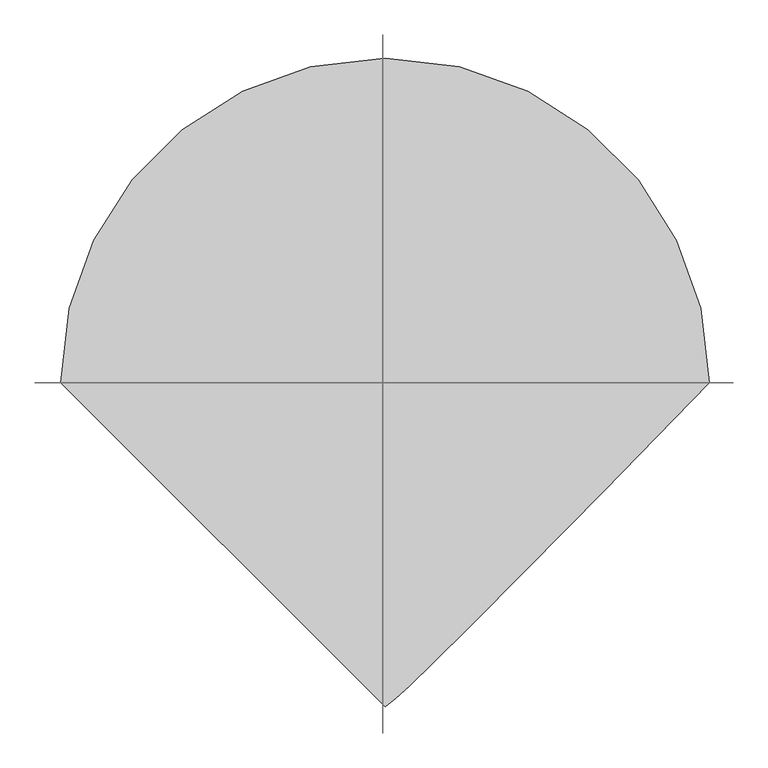
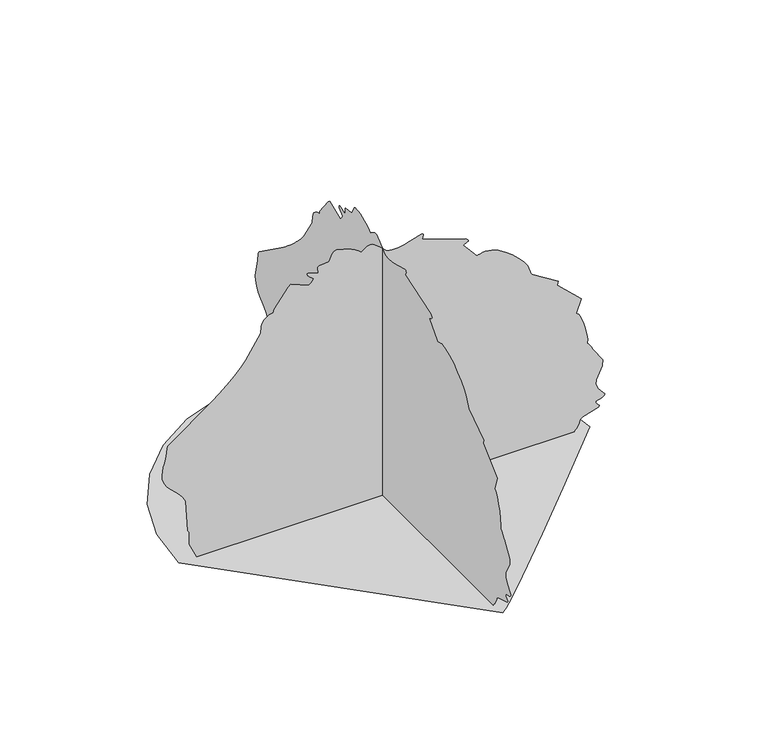
"""IFC4 building model written with IfcOpenShell, lengths in millimetres: proxy geometry, holly 26750 : holly 26750."""

from ifc_helpers import new_model, si_unit, origin, place, context, project, spatial, triangles, source, transform, mapped, element, save


def entourage_ccbe6d7c(model_context):
    return source(origin(), model_context, "Body", "Tessellation", [
        triangles([(-948.1489574, 0.0, 0.0001584), (-923.0842083, 217.2530545, 0.0001584), (-851.6949612, 416.7657311, 0.0001584), (-739.7012884, 592.8207553, 0.0001584), (-592.8207553, 739.7012884, 0.0001584), (-416.7657311, 851.6949612, 0.0001584), (-217.2530545, 923.0816648, 0.0001584), (4.14e-05, 948.1489574, 0.0001584), (217.2530545, 923.0842083, 0.0001584), (416.7657311, 851.6949612, 0.0001584), (592.8207553, 739.7012884, 0.0001584), (739.7012884, 592.8207553, 0.0001584), (851.6949612, 416.7657311, 0.0001584), (923.0816648, 217.2530545, 0.0001584), (948.1489574, -8.29e-05, 0.0001584), (640.0215443, -316.0623576, 0.0001584), (411.5917374, -548.7669763, 0.0001584), (249.5753185, -712.0026157, 0.0001584), (140.6913579, -819.6655935, 0.0001584), (71.6559369, -885.64972, 0.0001584), (29.1863771, -923.8462257, 0.0001584), (-0.0001243, -948.1489574, 0.0001584), (-7.5086714, 195.1763861, 1267.2389282), (-7.5086714, 179.2483067, 1263.2994884), (-7.5086714, 162.0304078, 1257.8307816), (-7.5086714, 144.4787539, 1250.7569401), (-7.5086714, 127.5514259, 1242.0092182), (-7.5086714, 112.2047518, 1231.5139286), (-7.5086714, 99.3960405, 1219.1973839), (-7.5086714, 96.3241623, 1220.6731659), (-7.5086714, 91.1522123, 1224.4323841), (-7.5086714, 84.5334848, 1229.4921043), (-7.5086714, 77.1194751, 1234.8564571), (-7.5086714, 69.5642495, 1239.5377121), (-7.5086714, 62.5195578, 1242.5399998), (-7.5086714, 56.6381899, 1242.880386), (-7.5086714, 48.1497636, 1241.0642178), (-7.5086714, 38.0075433, 1235.3112259), (-7.5086714, 26.6616175, 1226.6954727), (-7.5086714, 14.5605495, 1216.2942181), (-7.5086714, 2.1549868, 1205.1816696), (-7.5086714, -10.1063292, 1194.4323984), (-7.5086714, -21.7735642, 1185.1233009), (-7.5086714, -44.9310738, 1181.1406225), (-7.5086714, -71.2939859, 1182.9871668), (-7.5086714, -98.7844045, 1188.6996088), (-7.5086714, -125.3246087, 1196.3018337), (-7.5086714, -178.4657237, 1210.777331), (-7.5086714, -184.0044481, 1210.1194496), (-7.5086714, -186.6691655, 1206.9444254), (-7.5086714, -187.1967314, 1202.1768385), (-7.5086714, -182.6755321, 1185.5170269), (-7.5086714, -383.1462716, 1117.5161631), (-7.5086714, -393.1767277, 1109.7361147), (-7.5086714, -395.0157143, 1105.6136919), (-7.5086714, -393.8879488, 1102.1694254), (-7.5086714, -390.6062814, 1099.2180067), (-7.5086714, -372.1277581, 1088.6871088), (-7.5086714, -435.2772466, 1017.1175674), (-7.5086714, -437.7283324, 1017.437606), (-7.5086714, -442.2698793, 1018.3037596), (-7.5086714, -448.2439333, 1019.5610229), (-7.5086714, -454.9825481, 1021.0621668), (-7.5086714, -461.822792, 1022.6598164), (-7.5086714, -468.1067471, 1024.2016554), (-7.5086714, -473.166431, 1025.537693), (-7.5086714, -502.5059555, 1020.5592905), (-7.5086714, -534.2381756, 1007.0464525), (-7.5086714, -566.6435014, 987.1252121), (-7.5086714, -598.0048865, 962.9266891), (-7.5086714, -626.6103716, 936.5792421), (-7.5086714, -650.7352798, 910.2089767), (-7.5086714, -668.6702316, 885.9468676), (-7.5086714, -686.5644882, 838.1898262), (-7.5086714, -809.9704004, 760.305772), (-7.5086714, -805.7591022, 743.4655935), (-7.5086714, -915.2203714, 638.2130791), (-7.5086714, -894.1714382, 575.0635906), (-7.5086714, -903.617664, 567.5579078), (-7.5086714, -914.1053232, 547.8068604), (-7.5086714, -924.5625338, 519.9684434), (-7.5086714, -933.9198841, 488.2006877), (-7.5086714, -941.1080355, 456.6564285), (-7.5086714, -945.0552509, 429.4962041), (-7.5086714, -944.6894302, 410.8729222), (-7.5086714, -947.6840876, 408.4091191), (-7.5086714, -951.631303, 403.9311221), (-7.5086714, -956.0813948, 398.0789357), (-7.5086714, -960.5872971, 391.4952533), (-7.5086714, -964.7020895, 384.820152), (-7.5086714, -967.971076, 378.6987597), (-7.5086714, -969.9497343, 373.7711535), (-7.5086714, -1015.9974323, 304.568855), (-7.5086714, -1014.0136871, 276.7279126), (-7.5086714, -984.4354053, 218.9253907), (-7.5086714, -983.4092325, 198.3142941), (-7.5086714, -995.1541552, 172.0712739), (-7.5086714, -1024.6817133, 137.2212117), (-7.5086714, -1022.9417759, 130.8493623), (-7.5086714, -1018.3139334, 126.0055809), (-7.5086714, -1011.6743677, 122.4462869), (-7.5086714, -982.5811581, 116.1709614), (-7.5086714, -982.5024565, 110.3304839), (-7.5086714, -984.7630743, 105.408982), (-7.5086714, -999.0657623, 90.4069817), (-7.5086714, -999.4214092, 86.700867), (-7.5086714, -994.9103474, 81.6175654), (-7.5086714, -922.3882479, 60.3801172), (-7.5086714, -911.0090733, 53.020719), (-7.5086714, -909.9524517, 45.2163171), (-7.5086714, -907.5597198, 37.5411996), (-7.5086714, -904.0596428, 29.9740312), (-7.5086714, -899.6679777, 22.4928926), (-7.5086714, -894.6082575, 15.0766517), (-7.5086714, -889.1066311, 7.7034389), (-7.5086714, -883.3814718, 0.3517747), (-7.5086714, 857.0696331, 0.0), (-7.5086714, 890.8821041, 74.070715), (-7.5086714, 890.8821041, 133.011158), (-7.5086714, 897.8544256, 142.0888652), (-7.5086714, 906.9323599, 288.2569691), (-7.5086714, 918.2785423, 310.329568), (-7.5086714, 934.7885084, 330.547956), (-7.5086714, 954.1814381, 349.7579753), (-7.5086714, 974.171279, 368.8105187), (-7.5086714, 992.4846233, 388.5513923), (-7.5086714, 1006.8356369, 409.831525), (-7.5086714, 1014.945825, 433.5017735), (-7.5086714, 1016.3835279, 454.0351496), (-7.5086714, 1014.4251446, 473.0826061), (-7.5086714, 1010.2722731, 490.9768991), (-7.5086714, 1005.1338512, 508.0558711), (-7.5086714, 996.7289864, 541.0987307), (-7.5086714, 993.7038076, 576.6841312), (-7.5086714, 989.7007816, 586.0592494), (-7.5086714, 986.7239285, 589.1733035), (-7.5086714, 784.7202702, 733.315777), (-7.5086714, 753.8211388, 759.3609169), (-7.5086714, 719.0663561, 789.2566938), (-7.5086714, 684.3724709, 820.8568726), (-7.5086714, 653.6486195, 852.0099129), (-7.5086714, 630.8089525, 880.5697248), (-7.5086714, 562.4982239, 987.6459652), (-7.5086714, 559.6966144, 1020.7294109), (-7.5086714, 555.292232, 1034.4301735), (-7.5086714, 548.0761027, 1046.0812065), (-7.5086714, 537.4512789, 1055.5756851), (-7.5086714, 522.8132552, 1062.7994448), (-7.5086714, 503.5575265, 1067.6381756), (-7.5086714, 500.3495101, 1081.6894255), (-7.5086714, 435.3305863, 1167.4931997), (-7.5086714, 423.5678596, 1177.0969013), (-7.5086714, 339.3668581, 1143.4165443), (-7.5086714, 336.5372706, 1144.8643484), (-7.5086714, 333.0320704, 1147.7802315), (-7.5086714, 329.2195487, 1151.7172005), (-7.5086714, 318.3178522, 1168.6768484), (-7.5086714, 338.9502774, 1184.7296476), (-7.5086714, 344.6017857, 1191.1278763), (-7.5086714, 347.962191, 1197.2136967), (-7.5086714, 347.7869473, 1202.3572054), (-7.5086714, 343.1539816, 1204.0539042), (-7.5086714, 297.2663574, 1189.7283251), (-7.5086714, 299.3516952, 1212.9287258), (-7.5086714, 298.767483, 1216.5431128), (-7.5086714, 297.2663574, 1219.1973839), (-7.5086714, 292.6613332, 1221.3539383), (-7.5086714, 249.2443431, 1226.9900768), (-7.5086714, 246.747021, 1227.6175095), (-7.5086714, 231.2268564, 1258.3413609), (-7.5086714, 224.3381235, 1265.7124226), (-7.5086714, 216.7902557, 1269.9999516), (-7.5086714, 208.8568192, 1269.717992), (-202.6848849, 7.94e-05, 1267.2389282), (-186.7567873, 7.9e-05, 1263.2994884), (-169.5388885, 7.87e-05, 1257.8307816), (-151.9872436, 7.84e-05, 1250.7569401), (-135.0599247, 7.8e-05, 1242.0092182), (-119.7134959, 7.75e-05, 1231.5139286), (-106.9047846, 7.68e-05, 1219.1973839), (-103.8329063, 7.69e-05, 1220.6731659), (-98.6609655, 7.7e-05, 1224.4323841), (-92.0419745, 7.73e-05, 1229.4921043), (-84.6279739, 7.75e-05, 1234.8564571), (-77.0729936, 7.78e-05, 1239.5377121), (-70.0280521, 7.8e-05, 1242.5399998), (-64.1469339, 7.83e-05, 1242.880386), (-55.6582578, 7.75e-05, 1241.0642178), (-45.5160353, 7.69e-05, 1235.3112259), (-34.1701118, 7.64e-05, 1226.6954727), (-22.0691448, 7.6e-05, 1216.2942181), (-9.6635817, 7.56e-05, 1205.1816696), (2.5977342, 7.53e-05, 1194.4323984), (14.26497, 7.48e-05, 1185.1233009), (37.4223274, 7.46e-05, 1181.1406225), (63.7852418, 7.46e-05, 1182.9871668), (91.2759148, 7.49e-05, 1188.6996088), (117.816119, 7.54e-05, 1196.3018337), (170.9569705, 7.63e-05, 1210.777331), (176.4956949, 7.62e-05, 1210.1194496), (179.1604124, 7.6e-05, 1206.9444254), (179.6879783, 7.57e-05, 1202.1768385), (175.1670333, 7.48e-05, 1185.5170269), (375.6380453, 7.06e-05, 1117.5161631), (385.6685014, 7.03e-05, 1109.7361147), (387.5074516, 7.02e-05, 1105.6136919), (386.3797225, 7e-05, 1102.1694254), (383.0980187, 6.98e-05, 1099.2180067), (364.6195318, 6.91e-05, 1088.6871088), (427.7690203, 6.48e-05, 1017.1175674), (430.2201061, 6.48e-05, 1017.437606), (434.7616167, 6.49e-05, 1018.3037596), (440.735707, 6.5e-05, 1019.5610229), (447.4743218, 6.5e-05, 1021.0621668), (454.3145293, 6.51e-05, 1022.6598164), (460.5984844, 6.52e-05, 1024.2016554), (465.6581683, 6.53e-05, 1025.537693), (494.9977292, 6.5e-05, 1020.5592905), (526.7299493, 6.42e-05, 1007.0464525), (559.1352751, 6.3e-05, 987.1252121), (590.4966239, 6.16e-05, 962.9266891), (619.0995655, 6e-05, 936.5792421), (643.2270172, 5.84e-05, 910.2089767), (661.161969, 5.7e-05, 885.9468676), (679.0537548, 5.41e-05, 838.1898262), (802.4621378, 4.95e-05, 760.305772), (798.2508396, 4.85e-05, 743.4655935), (907.7121815, 4.22e-05, 638.2156225), (886.6606321, 3.85e-05, 575.0635906), (896.1094013, 3.8e-05, 567.5579078), (906.5970606, 3.68e-05, 547.8068604), (917.0542711, 3.52e-05, 519.9684434), (926.4116215, 3.33e-05, 488.2006877), (933.5973021, 3.14e-05, 456.6564285), (937.5444448, 2.98e-05, 429.4962041), (937.1812403, 2.87e-05, 410.8729222), (940.1758976, 2.85e-05, 408.4091191), (944.1230404, 2.83e-05, 403.9311221), (948.5731321, 2.79e-05, 398.0789357), (953.0791071, 2.75e-05, 391.4952533), (957.1913561, 2.71e-05, 384.820152), (960.462886, 2.68e-05, 378.6987597), (962.4415443, 2.65e-05, 373.7711535), (1008.4891697, 2.23e-05, 304.568855), (1006.5054245, 2.07e-05, 276.7279126), (976.9271427, 1.72e-05, 218.9253907), (975.9009699, 1.6e-05, 198.3142941), (987.6459652, 1.44e-05, 172.0712739), (1017.1734507, 1.24e-05, 137.2212117), (1015.4335133, 1.2e-05, 130.8493623), (1010.8056707, 1.17e-05, 126.0058353), (1004.1661051, 1.15e-05, 122.4462869), (975.0729681, 1.11e-05, 116.1712157), (974.9941938, 1.11e-05, 110.3304839), (977.2548117, 1.08e-05, 105.408982), (991.5575724, 9.4e-06, 90.407236), (991.9131466, 9.3e-06, 86.700867), (987.4020847, 9.1e-06, 81.6175654), (914.8800579, 7.5e-06, 60.3801172), (903.5008106, 7.3e-06, 53.020719), (902.4441891, 7.5e-06, 45.2163171), (900.0515299, 7.5e-06, 37.5411996), (896.5488367, 7.3e-06, 29.9740312), (892.1597151, 6.9e-06, 22.4929448), (887.1000675, 6.5e-06, 15.0767278), (881.5984411, 6e-06, 7.7034894), (875.8732819, 5.5e-06, 0.3518408), (-864.5778957, 4.1e-06, 6.72e-05), (-898.3903667, 8.6e-06, 74.0709693), (-898.3903667, 1.21e-05, 133.011158), (-905.3626156, 1.26e-05, 142.0888652), (-914.4406225, 2.14e-05, 288.2569691), (-925.7893484, 2.27e-05, 310.3321115), (-942.296771, 2.39e-05, 330.547956), (-961.6897007, 2.5e-05, 349.7579753), (-981.6820124, 2.62e-05, 368.8105187), (-999.992886, 2.73e-05, 388.5513923), (-1014.3438995, 2.86e-05, 409.831525), (-1022.4540876, 3e-05, 433.5017735), (-1023.8917179, 3.12e-05, 454.0351496), (-1021.9334072, 3.24e-05, 473.0826061), (-1017.7805357, 3.34e-05, 490.9768991), (-1012.6421139, 3.45e-05, 508.0558711), (-1004.237249, 3.64e-05, 541.0987307), (-1001.2146137, 3.86e-05, 576.6841312), (-997.2090443, 3.92e-05, 586.0592494), (-994.2347345, 3.94e-05, 589.1733035), (-792.2285328, 4.83e-05, 733.315777), (-761.3294014, 5.01e-05, 759.3609169), (-726.5746187, 5.21e-05, 789.2566938), (-691.8807335, 5.41e-05, 820.8568726), (-661.1568821, 5.59e-05, 852.0099129), (-638.3172152, 5.74e-05, 880.5697248), (-570.0064502, 6.3e-05, 987.6459652), (-567.2048407, 6.5e-05, 1020.7294109), (-562.8004947, 6.58e-05, 1034.4301735), (-555.584329, 6.65e-05, 1046.0812065), (-544.9595052, 6.71e-05, 1055.5756851), (-530.3215178, 6.75e-05, 1062.7994448), (-511.0682962, 6.78e-05, 1067.6381756), (-507.8577364, 6.87e-05, 1081.6894255), (-442.8413561, 7.38e-05, 1167.4931997), (-431.0760859, 7.43e-05, 1177.0969013), (-346.8750844, 7.23e-05, 1143.4165443), (-344.0455333, 7.24e-05, 1144.8643484), (-340.540333, 7.26e-05, 1147.7802315), (-336.727775, 7.28e-05, 1151.7172005), (-325.8261148, 7.38e-05, 1168.6768484), (-346.4585401, 7.48e-05, 1184.7296476), (-352.110012, 7.51e-05, 1191.1278763), (-355.4704536, 7.55e-05, 1197.2136967), (-355.2951736, 7.58e-05, 1202.3572054), (-350.6622442, 7.57e-05, 1204.0539042), (-304.7771271, 7.51e-05, 1189.7283251), (-306.8599397, 7.63e-05, 1212.9287258), (-306.2757457, 7.65e-05, 1216.5431128), (-304.7771271, 7.68e-05, 1219.1973839), (-300.1695595, 7.68e-05, 1221.3539383), (-256.7533506, 7.73e-05, 1226.9900768), (-254.2565372, 7.74e-05, 1227.6175095), (-238.7353552, 7.86e-05, 1258.3413609), (-231.8468767, 7.9e-05, 1265.7124226), (-224.2990089, 7.94e-05, 1269.9999516), (-216.3655724, 7.99e-05, 1269.717992)], [[22, 21, 1], [21, 20, 1], [20, 19, 1], [19, 18, 1], [18, 17, 1], [1, 17, 2], [2, 17, 3], [3, 17, 4], [17, 16, 4], [4, 16, 5], [5, 16, 6], [6, 16, 7], [7, 16, 8], [8, 16, 9], [9, 16, 10], [10, 16, 11], [11, 16, 12], [16, 15, 12], [15, 14, 12], [14, 13, 12], [75, 74, 76], [161, 160, 162], [117, 116, 118], [118, 116, 119], [77, 76, 78], [160, 159, 162], [159, 158, 162], [158, 157, 162], [162, 157, 163], [152, 151, 153], [116, 115, 119], [115, 114, 119], [114, 113, 119], [113, 112, 119], [112, 111, 119], [111, 110, 119], [110, 109, 119], [98, 97, 99], [99, 97, 100], [100, 97, 101], [101, 97, 102], [119, 109, 120], [120, 109, 121], [121, 109, 122], [106, 105, 107], [105, 104, 107], [107, 104, 108], [104, 103, 108], [151, 150, 153], [150, 149, 153], [49, 48, 50], [50, 48, 51], [51, 48, 52], [48, 47, 52], [122, 109, 123], [55, 54, 56], [56, 54, 57], [54, 53, 57], [57, 53, 58], [53, 52, 58], [109, 108, 123], [103, 102, 108], [93, 92, 94], [94, 92, 95], [97, 96, 102], [102, 96, 108], [108, 96, 123], [96, 95, 123], [95, 92, 123], [92, 91, 123], [91, 90, 123], [90, 89, 123], [89, 88, 123], [88, 87, 123], [87, 86, 123], [86, 85, 123], [85, 84, 123], [84, 83, 123], [83, 82, 123], [82, 81, 123], [81, 80, 123], [80, 79, 123], [79, 78, 123], [78, 76, 123], [76, 74, 123], [74, 73, 123], [73, 72, 123], [72, 71, 123], [71, 70, 123], [70, 69, 123], [69, 68, 123], [68, 67, 123], [67, 66, 123], [66, 65, 123], [65, 64, 123], [64, 63, 123], [63, 62, 123], [62, 61, 123], [61, 60, 123], [60, 59, 123], [59, 58, 123], [58, 52, 123], [52, 47, 123], [47, 46, 123], [46, 45, 123], [45, 44, 123], [44, 43, 123], [43, 42, 123], [42, 41, 123], [41, 40, 123], [40, 39, 123], [39, 38, 123], [38, 37, 123], [37, 36, 123], [36, 35, 123], [35, 34, 123], [34, 33, 123], [33, 32, 123], [32, 31, 123], [31, 30, 123], [30, 29, 123], [123, 29, 124], [29, 28, 124], [28, 27, 124], [27, 26, 124], [26, 25, 124], [25, 24, 124], [24, 23, 124], [23, 173, 124], [124, 173, 125], [125, 173, 126], [166, 165, 167], [165, 164, 167], [164, 163, 167], [167, 163, 168], [172, 171, 173], [171, 170, 173], [170, 169, 173], [173, 169, 126], [169, 168, 126], [126, 168, 127], [127, 168, 128], [128, 168, 129], [129, 168, 130], [130, 168, 131], [131, 168, 132], [146, 145, 147], [147, 145, 148], [145, 144, 148], [148, 144, 149], [144, 143, 149], [149, 143, 153], [143, 142, 153], [135, 134, 136], [134, 133, 136], [136, 133, 137], [133, 132, 137], [153, 142, 154], [157, 156, 163], [163, 156, 168], [142, 141, 154], [137, 132, 138], [138, 132, 139], [154, 141, 155], [141, 140, 155], [156, 155, 168], [168, 155, 132], [155, 140, 132], [132, 140, 139], [226, 225, 227], [312, 311, 313], [268, 267, 269], [269, 267, 270], [228, 227, 229], [311, 310, 313], [310, 309, 313], [309, 308, 313], [313, 308, 314], [303, 302, 304], [267, 266, 270], [266, 265, 270], [265, 264, 270], [264, 263, 270], [263, 262, 270], [262, 261, 270], [261, 260, 270], [249, 248, 250], [250, 248, 251], [251, 248, 252], [252, 248, 253], [270, 260, 271], [271, 260, 272], [272, 260, 273], [257, 256, 258], [256, 255, 258], [258, 255, 259], [255, 254, 259], [302, 301, 304], [301, 300, 304], [200, 199, 201], [201, 199, 202], [202, 199, 203], [199, 198, 203], [273, 260, 274], [206, 205, 207], [207, 205, 208], [205, 204, 208], [208, 204, 209], [204, 203, 209], [260, 259, 274], [254, 253, 259], [244, 243, 245], [245, 243, 246], [248, 247, 253], [253, 247, 259], [259, 247, 274], [247, 246, 274], [246, 243, 274], [243, 242, 274], [242, 241, 274], [241, 240, 274], [240, 239, 274], [239, 238, 274], [238, 237, 274], [237, 236, 274], [236, 235, 274], [235, 234, 274], [234, 233, 274], [233, 232, 274], [232, 231, 274], [231, 230, 274], [230, 229, 274], [229, 227, 274], [227, 225, 274], [225, 224, 274], [224, 223, 274], [223, 222, 274], [222, 221, 274], [221, 220, 274], [220, 219, 274], [219, 218, 274], [218, 217, 274], [217, 216, 274], [216, 215, 274], [215, 214, 274], [214, 213, 274], [213, 212, 274], [212, 211, 274], [211, 210, 274], [210, 209, 274], [209, 203, 274], [203, 198, 274], [198, 197, 274], [197, 196, 274], [196, 195, 274], [195, 194, 274], [194, 193, 274], [193, 192, 274], [192, 191, 274], [191, 190, 274], [190, 189, 274], [189, 188, 274], [188, 187, 274], [187, 186, 274], [186, 185, 274], [185, 184, 274], [184, 183, 274], [183, 182, 274], [182, 181, 274], [181, 180, 274], [274, 180, 275], [180, 179, 275], [179, 178, 275], [178, 177, 275], [177, 176, 275], [176, 175, 275], [175, 174, 275], [174, 324, 275], [275, 324, 276], [276, 324, 277], [317, 316, 318], [316, 315, 318], [315, 314, 318], [318, 314, 319], [323, 322, 324], [322, 321, 324], [321, 320, 324], [324, 320, 277], [320, 319, 277], [277, 319, 278], [278, 319, 279], [279, 319, 280], [280, 319, 281], [281, 319, 282], [282, 319, 283], [297, 296, 298], [298, 296, 299], [296, 295, 299], [299, 295, 300], [295, 294, 300], [300, 294, 304], [294, 293, 304], [286, 285, 287], [285, 284, 287], [287, 284, 288], [284, 283, 288], [304, 293, 305], [308, 307, 314], [314, 307, 319], [293, 292, 305], [288, 283, 289], [289, 283, 290], [305, 292, 306], [292, 291, 306], [307, 306, 319], [319, 306, 283], [306, 291, 283], [283, 291, 290]], closed=False),
    ])


if __name__ == "__main__":
    model = new_model("IFC4")
    model_context = context("Model", 3, world=origin())
    ifc_project = project(units=[si_unit("LENGTHUNIT", "METRE", prefix="MILLI")], contexts=[model_context])
    site = spatial("IfcSite", under=ifc_project)
    building = spatial("IfcBuilding", under=site)
    placement = place(None, origin())
    entourage_shape = entourage_ccbe6d7c(model_context)
    element("IfcBuildingElementProxy", 1, Name="holly 26750 : holly 26750", ObjectType="holly 26750 : holly 26750", at=placement, inside=building, context=model_context, shape_type="MappedRepresentation", body=[
        mapped(entourage_shape, transform((0.0, 0.0, 0.0), x_axis=(1.0, 0.0, 0.0), y_axis=(0.0, 1.0, 0.0), z_axis=(0.0, 0.0, 1.0))),
    ])
    save(model, "model.ifc")

# Revit data of these elements
# Type "holly 26750 : holly 26750"
#   built-in parameter 1005195 = "RPC-16-FVGN-EMQ0-7PXJ-Q000-ST1L-LVER-AU"
#   Height = 0
